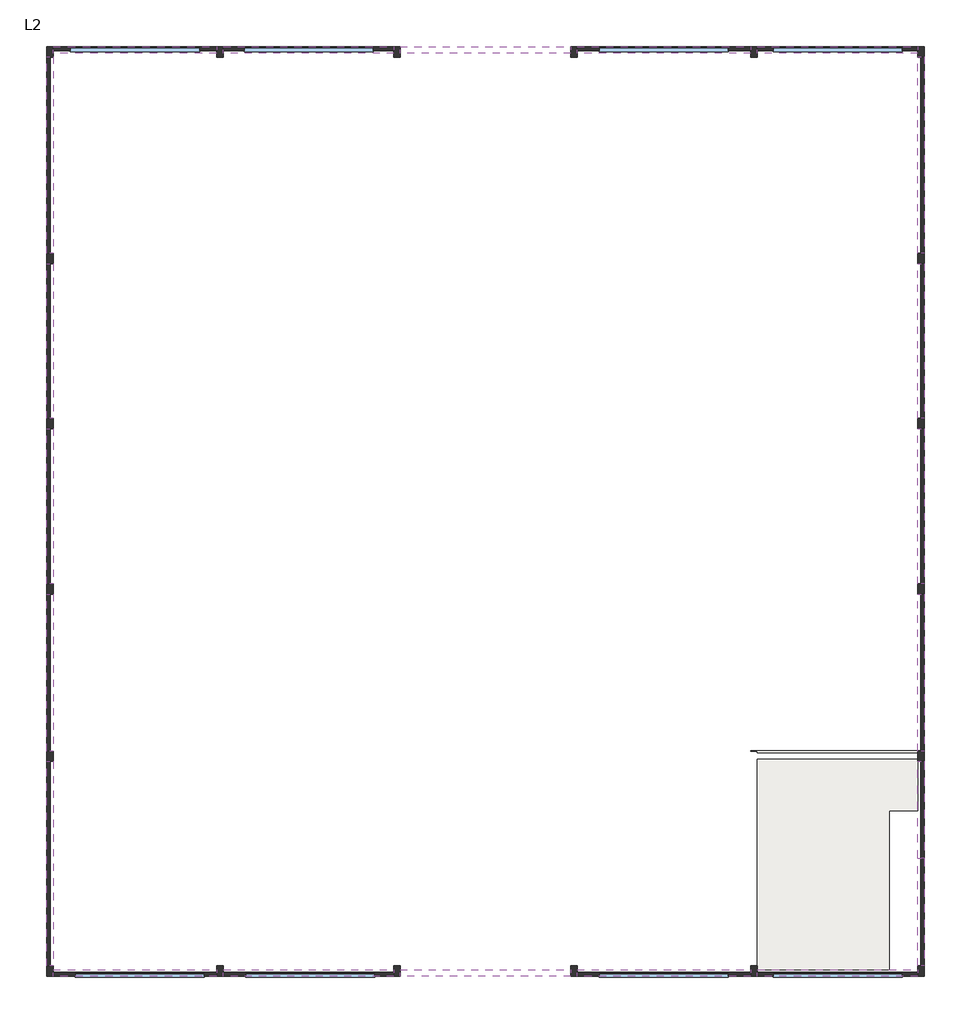
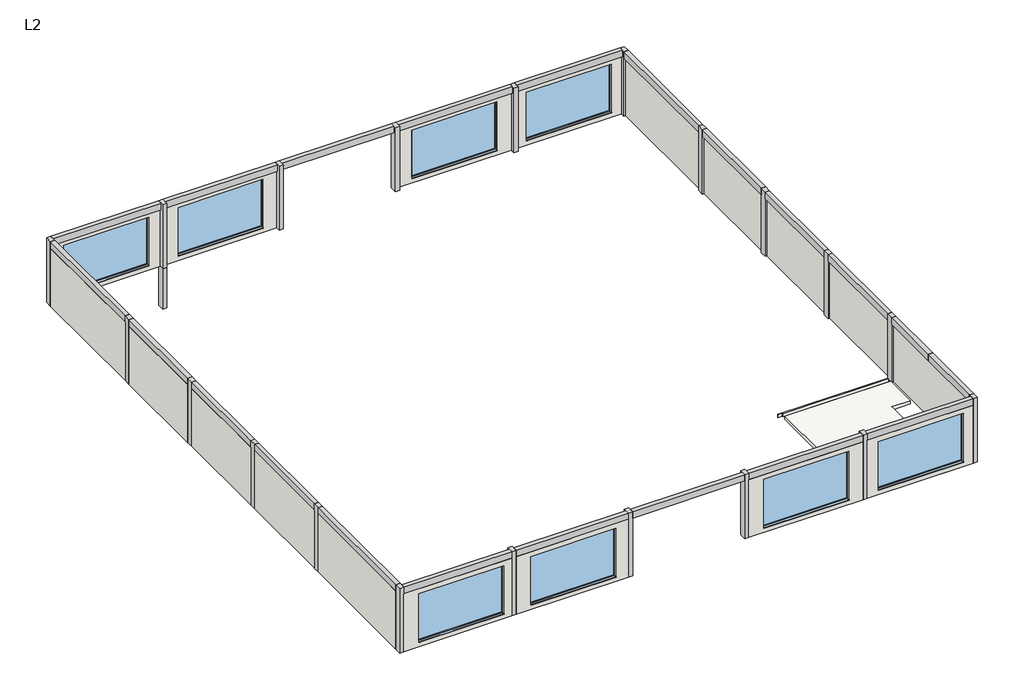
# One storey: 21 beams, 21 columns, 18 walls, 8 windows, 1 slab.
"""IFC4 building model written with IfcOpenShell, lengths in millimetres."""

import ifcopenshell
import ifcopenshell.guid

model = None  # the IFC model being written
_history = None  # IfcOwnerHistory: only IFC2X3 demands one
_inside = {}  # id of a spatial element -> (the spatial element, [elements in it])
_under = {}  # id of a project, library or spatial element -> (it, [spatial elements below it])
_declared = {}  # id of a project -> (the project, [libraries it declares])
_typed = {}  # id of a type object -> (the type object, [elements of that type])
_made_of = {}  # id of a material, layer set ... -> (it, [elements and type objects made of it])


def new_model(schema):
    """Start an empty IFC model of exactly this schema.

    Asked for "IFC4X3", IfcOpenShell would pick the latest addendum, in which some entities
    have other attributes; the version numbers below select the first issue.
    IFC2X3 requires an IfcOwnerHistory on every rooted entity: one is made here for all.
    """
    global model, _history
    if schema == "IFC4X3":
        model = ifcopenshell.file(schema_version=(4, 3, 0, 0))
    else:
        model = ifcopenshell.file(schema=schema)
    _inside.clear()
    _under.clear()
    _declared.clear()
    _typed.clear()
    _made_of.clear()
    _history = None
    if model.schema == "IFC2X3":
        org = make("IfcOrganization", Name="unknown")
        user = make(
            "IfcPersonAndOrganization",
            ThePerson=make("IfcPerson", FamilyName="unknown"),
            TheOrganization=org,
        )
        app = make(
            "IfcApplication",
            ApplicationDeveloper=org,
            Version="unknown",
            ApplicationFullName="unknown",
            ApplicationIdentifier="unknown",
        )
        _history = make(
            "IfcOwnerHistory",
            OwningUser=user,
            OwningApplication=app,
            ChangeAction="ADDED",
            CreationDate=0,
        )
    return model


def make(cls, **values):
    """One entity of the class cls with the attributes given. An attribute that is None is left unset."""
    return model.create_entity(
        cls, **{name: value for name, value in values.items() if value is not None}
    )


def rooted(cls, **values):
    """An entity with a GlobalId (a new one), such as an element, a storey or a relation."""
    return make(cls, GlobalId=ifcopenshell.guid.new(), OwnerHistory=_history, **values)


def si_unit(unit_type, name, prefix=None):
    """IfcSIUnit, for example si_unit("LENGTHUNIT", "METRE", prefix="MILLI")."""
    return make("IfcSIUnit", UnitType=unit_type, Prefix=prefix, Name=name)


def assignment(units):
    """IfcUnitAssignment: the units of a project."""
    return None if units is None else make("IfcUnitAssignment", Units=units)


def point(xyz):
    """IfcCartesianPoint."""
    return None if xyz is None else make("IfcCartesianPoint", Coordinates=xyz)


def direction(xyz):
    """IfcDirection."""
    return None if xyz is None else make("IfcDirection", DirectionRatios=xyz)


def frame(location, z_axis=None, x_axis=None):
    """IfcAxis2Placement3D, a coordinate frame: its origin and axes. An axis left out is left unset."""
    return make(
        "IfcAxis2Placement3D",
        Location=point(location),
        Axis=direction(z_axis),
        RefDirection=direction(x_axis),
    )


def origin():
    """The frame at (0, 0, 0) with its axes left unset."""
    return frame((0.0, 0.0, 0.0))


def place(relative_to, where):
    """IfcLocalPlacement: puts the frame where relative to a parent placement (None: the world)."""
    return make(
        "IfcLocalPlacement", PlacementRelTo=relative_to, RelativePlacement=where
    )


def context(
    kind, dimensions, precision=None, world=None, true_north=None, identifier=None
):
    """IfcGeometricRepresentationContext, for example the 3D "Model" context."""
    return make(
        "IfcGeometricRepresentationContext",
        ContextIdentifier=identifier,
        ContextType=kind,
        CoordinateSpaceDimension=dimensions,
        Precision=precision,
        WorldCoordinateSystem=world,
        TrueNorth=true_north,
    )


def project(units=None, contexts=None):
    """IfcProject with its units and contexts."""
    return rooted(
        "IfcProject",
        Name="project",
        RepresentationContexts=contexts,
        UnitsInContext=assignment(units),
    )


def spatial(cls, under=None, at=None, **own):
    """A site, building, storey or space (cls), placed at a placement, below another one or the project."""
    s = rooted(cls, ObjectPlacement=at, **own)
    if under is not None:
        _under.setdefault(under.id(), (under, []))[1].append(s)
    return s


def polyline(points):
    """IfcPolyline through the points."""
    return make("IfcPolyline", Points=[point(p) for p in points])


def outline(outer, holes=None, kind="AREA"):
    """IfcArbitraryClosedProfileDef: a profile drawn as a closed curve; with holes, ...WithVoids."""
    if holes is None:
        return make("IfcArbitraryClosedProfileDef", ProfileType=kind, OuterCurve=outer)
    return make(
        "IfcArbitraryProfileDefWithVoids",
        ProfileType=kind,
        OuterCurve=outer,
        InnerCurves=holes,
    )


def extrude(swept, where, along, depth):
    """IfcExtrudedAreaSolid: the profile swept, set in the frame where, extruded along a direction by depth."""
    return make(
        "IfcExtrudedAreaSolid",
        SweptArea=swept,
        Position=where,
        ExtrudedDirection=direction(along),
        Depth=depth,
    )


def faces_of(points, faces, orient=None, outer=None):
    """IfcFace entities. A face is a list of loops; a loop is a list of indices into points, from 0.

    orient and outer hold one flag for each loop. By default every Orientation is true, the
    first loop of a face is its IfcFaceOuterBound and the others are IfcFaceBound.
    """
    made = []
    for i, loops in enumerate(faces):
        bounds = []
        for j, loop in enumerate(loops):
            is_outer = j == 0 if outer is None else outer[i][j]
            bounds.append(
                make(
                    "IfcFaceOuterBound" if is_outer else "IfcFaceBound",
                    Bound=make("IfcPolyLoop", Polygon=[points[k] for k in loop]),
                    Orientation=True if orient is None else orient[i][j],
                )
            )
        made.append(make("IfcFace", Bounds=bounds))
    return made


def faceted_brep(points, faces, orient=None, outer=None, voids=None):
    """IfcFacetedBrep: a solid bounded by flat faces; with voids (closed shells), ...WithVoids."""
    shared = [point(p) for p in points]
    hull = make("IfcClosedShell", CfsFaces=faces_of(shared, faces, orient, outer))
    if voids is None:
        return make("IfcFacetedBrep", Outer=hull)
    return make(
        "IfcFacetedBrepWithVoids",
        Outer=hull,
        Voids=[
            make(cls, CfsFaces=faces_of(shared, fs, o, b)) for cls, fs, o, b in voids
        ],
    )


def shape(context_of_items, identifier, shape_type, items):
    """IfcShapeRepresentation: the items that make up one representation, for example the "Body"."""
    return make(
        "IfcShapeRepresentation",
        ContextOfItems=context_of_items,
        RepresentationIdentifier=identifier,
        RepresentationType=shape_type,
        Items=items,
    )


def source(mapping_origin, context_of_items, identifier, shape_type, items):
    """IfcRepresentationMap: a shape defined once, which mapped items show again and again."""
    return make(
        "IfcRepresentationMap",
        MappingOrigin=mapping_origin,
        MappedRepresentation=shape(context_of_items, identifier, shape_type, items),
    )


def transform(
    local_origin,
    x_axis=None,
    y_axis=None,
    z_axis=None,
    scale=None,
    scale2=None,
    scale3=None,
    uniform=True,
):
    """IfcCartesianTransformationOperator3D, or its non-uniform kind. x_axis, y_axis, z_axis: its Axis1, 2, 3."""
    if uniform:
        return make(
            "IfcCartesianTransformationOperator3D",
            Axis1=direction(x_axis),
            Axis2=direction(y_axis),
            LocalOrigin=point(local_origin),
            Scale=scale,
            Axis3=direction(z_axis),
        )
    return make(
        "IfcCartesianTransformationOperator3DnonUniform",
        Axis1=direction(x_axis),
        Axis2=direction(y_axis),
        LocalOrigin=point(local_origin),
        Scale=scale,
        Axis3=direction(z_axis),
        Scale2=scale2,
        Scale3=scale3,
    )


def mapped(mapping_source, mapping_target):
    """IfcMappedItem: shows the shape of a source again, moved by a transform."""
    return make(
        "IfcMappedItem", MappingSource=mapping_source, MappingTarget=mapping_target
    )


def made_of(thing, what):
    """Note that an element or type object is made of a material, layer set ...; save() writes the relation."""
    if what is not None:
        _made_of.setdefault(what.id(), (what, []))[1].append(thing)
    return thing


def element(
    cls,
    number,
    at=None,
    inside=None,
    cuts=None,
    type_object=None,
    material=None,
    context=None,
    identifier="Body",
    shape_type=None,
    held_by="IfcProductDefinitionShape",
    body=None,
    shapes=None,
    **own,
):
    """One element of the class cls, such as IfcWall. Its Tag is "e" and its number.

    at: its placement. inside: the storey or other place that contains it. cuts: it is an
    opening in that element (IfcRelVoidsElement). A single representation is given by context,
    identifier, shape_type and body (its items); several are given by shapes. held_by: the class
    of the entity that holds the representations. save() writes the other relations.
    """
    e = rooted(cls, Tag="e%d" % number, ObjectPlacement=at, **own)
    if body is not None:
        shapes = [shape(context, identifier, shape_type, body)]
    if shapes is not None:
        e.Representation = make(held_by, Representations=shapes)
    if inside is not None:
        _inside.setdefault(inside.id(), (inside, []))[1].append(e)
    if cuts is not None:
        rooted(
            "IfcRelVoidsElement", RelatingBuildingElement=cuts, RelatedOpeningElement=e
        )
    if type_object is not None:
        _typed.setdefault(type_object.id(), (type_object, []))[1].append(e)
    return made_of(e, material)


def aggregate(whole, parts):
    """IfcRelAggregates: a whole, such as a stair, and the parts it consists of."""
    return rooted("IfcRelAggregates", RelatingObject=whole, RelatedObjects=parts)


def save(model, path):
    """Write the relations noted so far, then the file.

    IfcRelAggregates (storeys below a building ...), IfcRelContainedInSpatialStructure (elements
    in a storey), IfcRelDefinesByType, IfcRelAssociatesMaterial and IfcRelDeclares: one each for
    every whole, place, type object, material and project.
    """
    for whole, parts in _under.values():
        aggregate(whole, parts)
    for where, things in _inside.values():
        rooted(
            "IfcRelContainedInSpatialStructure",
            RelatedElements=things,
            RelatingStructure=where,
        )
    for kind, things in _typed.values():
        rooted("IfcRelDefinesByType", RelatedObjects=things, RelatingType=kind)
    for what, things in _made_of.values():
        rooted("IfcRelAssociatesMaterial", RelatedObjects=things, RelatingMaterial=what)
    for by, libraries in _declared.values():
        rooted("IfcRelDeclares", RelatingContext=by, RelatedDefinitions=libraries)
    model.write(path)


def window_5000_x_3000mm_49c9fe68(model_context):
    return source(origin(), model_context, "Body", "SolidModel", [
        extrude(outline(polyline([(125.0, 920.0), (125.0, 900.0), (105.0, 900.0), (105.0, 910.0), (95.0, 910.0), (95.0, 900.0), (-25.0, 900.0), (-25.0, 920.0), (125.0, 920.0)])), frame((-2500.0, 0.0, 0.0), z_axis=(1.0, 0.0, 0.0), x_axis=(0.0, 1.0, 0.0)), (0.0, 0.0, 1.0), 5000.0),
        extrude(outline(polyline([(-2455.0, -49.0), (-2455.0, -35.0), (2455.0, -35.0), (2455.0, -49.0), (-2455.0, -49.0)])), frame((0.0, 0.0, 965.0), z_axis=(0.0, 0.0, 1.0), x_axis=(1.0, 0.0, 0.0)), (0.0, 0.0, 1.0), 2890.0),
        extrude(outline(polyline([(3865.0, -2465.0), (955.0, -2465.0), (955.0, 2465.0), (3865.0, 2465.0), (3865.0, -2465.0)]), holes=[polyline([(3840.0, 2440.0), (980.0, 2440.0), (980.0, -2440.0), (3840.0, -2440.0), (3840.0, 2440.0)])]), frame((0.0, -75.0, 0.0), z_axis=(0.0, 1.0, 0.0), x_axis=(0.0, 0.0, 1.0)), (0.0, 0.0, 1.0), 26.0),
        faceted_brep([(2500.0, -25.0, 3900.0), (2500.0, -75.0, 3900.0), (2500.0, -75.0, 900.0), (2500.0, -25.0, 900.0), (-2500.0, -75.0, 3900.0), (-2500.0, -75.0, 900.0), (-2465.0, -75.0, 3865.0), (2465.0, -75.0, 3865.0), (2465.0, -75.0, 955.0), (-2465.0, -75.0, 955.0), (-2500.0, -25.0, 900.0), (-2500.0, -25.0, 3900.0), (2440.0, -25.0, 3840.0), (-2440.0, -25.0, 3840.0), (-2440.0, -25.0, 980.0), (2440.0, -25.0, 980.0), (2440.0, -35.0, 3840.0), (2440.0, -35.0, 980.0), (-2440.0, -35.0, 980.0), (2465.0, -35.0, 3865.0), (-2465.0, -35.0, 3865.0), (-2465.0, -35.0, 955.0), (2465.0, -35.0, 955.0), (-2440.0, -35.0, 3840.0)], [[[0, 1, 2, 3]], [[2, 1, 4, 5], [6, 7, 8, 9]], [[5, 10, 3, 2]], [[10, 11, 0, 3], [12, 13, 14, 15]], [[16, 12, 15, 17]], [[17, 15, 14, 18]], [[19, 20, 21, 22], [23, 16, 17, 18]], [[7, 19, 22, 8]], [[8, 22, 21, 9]], [[13, 23, 18, 14]], [[20, 6, 9, 21]], [[4, 11, 10, 5]], [[11, 4, 1, 0]], [[23, 13, 12, 16]], [[6, 20, 19, 7]]]),
        extrude(outline(polyline([(3925.0, -2525.0), (875.0, -2525.0), (875.0, 2525.0), (3925.0, 2525.0), (3925.0, -2525.0)]), holes=[polyline([(3890.0, 2490.0), (910.0, 2490.0), (910.0, -2490.0), (3890.0, -2490.0), (3890.0, 2490.0)])]), frame((0.0, -80.0, 0.0), z_axis=(0.0, 1.0, 0.0), x_axis=(0.0, 0.0, 1.0)), (0.0, 0.0, 1.0), 5.0),
    ])


model = new_model("IFC4")

# Units and contexts
model_context = context("Model", 3, world=origin())
ifc_project = project(units=[si_unit("LENGTHUNIT", "METRE", prefix="MILLI")], contexts=[model_context])

# Site, building, storey
site = spatial("IfcSite", under=ifc_project)
building = spatial("IfcBuilding", under=site)
storey = spatial("IfcBuildingStorey", under=building, Name="L2", Elevation=4000.0)

# Beams
placement = place(None, origin())
element("IfcBeam", 1, ObjectType="M_Hormigón-Viga rectangular : 250 x 400mm", at=placement, inside=storey, context=model_context, shape_type="SweptSolid", body=[
    extrude(outline(polyline([(10525.0, 17750.0), (10525.0, 18000.0), (16750.0, 18000.0), (16750.0, 17750.0), (10525.0, 17750.0)])), frame((0.0, 0.0, 7600.0), z_axis=(0.0, 0.0, 1.0), x_axis=(1.0, 0.0, 0.0)), (0.0, 0.0, 1.0), 400.0),
])
element("IfcBeam", 2, ObjectType="M_Hormigón-Viga rectangular : 250 x 400mm", at=placement, inside=storey, context=model_context, shape_type="SweptSolid", body=[
    extrude(outline(polyline([(3550.0, 17750.0), (3550.0, 18000.0), (10275.0, 18000.0), (10275.0, 17750.0), (3550.0, 17750.0)])), frame((0.0, 0.0, 7600.0), z_axis=(0.0, 0.0, 1.0), x_axis=(1.0, 0.0, 0.0)), (0.0, 0.0, 1.0), 400.0),
])
element("IfcBeam", 3, ObjectType="M_Hormigón-Viga rectangular : 250 x 400mm", at=placement, inside=storey, context=model_context, shape_type="SweptSolid", body=[
    extrude(outline(polyline([(-3300.0, 17750.0), (-3300.0, 18000.0), (3300.0, 18000.0), (3300.0, 17750.0), (-3300.0, 17750.0)])), frame((0.0, 0.0, 7600.0), z_axis=(0.0, 0.0, 1.0), x_axis=(1.0, 0.0, 0.0)), (0.0, 0.0, 1.0), 400.0),
])
element("IfcBeam", 4, ObjectType="M_Hormigón-Viga rectangular : 250 x 400mm", at=placement, inside=storey, context=model_context, shape_type="SweptSolid", body=[
    extrude(outline(polyline([(-10150.0, 17750.0), (-10150.0, 18000.0), (-3550.0, 18000.0), (-3550.0, 17750.0), (-10150.0, 17750.0)])), frame((0.0, 0.0, 7600.0), z_axis=(0.0, 0.0, 1.0), x_axis=(1.0, 0.0, 0.0)), (0.0, 0.0, 1.0), 400.0),
])
element("IfcBeam", 5, ObjectType="M_Hormigón-Viga rectangular : 250 x 400mm", at=placement, inside=storey, context=model_context, shape_type="SweptSolid", body=[
    extrude(outline(polyline([(-16750.0, 17750.0), (-16750.0, 18000.0), (-10400.0, 18000.0), (-10400.0, 17750.0), (-16750.0, 17750.0)])), frame((0.0, 0.0, 7600.0), z_axis=(0.0, 0.0, 1.0), x_axis=(1.0, 0.0, 0.0)), (0.0, 0.0, 1.0), 400.0),
])
element("IfcBeam", 6, ObjectType="M_Hormigón-Viga rectangular : 250 x 400mm", at=placement, inside=storey, context=model_context, shape_type="SweptSolid", body=[
    extrude(outline(polyline([(16750.0, -17750.0), (16750.0, -18000.0), (10525.0, -18000.0), (10525.0, -17750.0), (16750.0, -17750.0)])), frame((0.0, 0.0, 7600.0), z_axis=(0.0, 0.0, 1.0), x_axis=(1.0, 0.0, 0.0)), (0.0, 0.0, 1.0), 400.0),
])
element("IfcBeam", 7, ObjectType="M_Hormigón-Viga rectangular : 250 x 400mm", at=placement, inside=storey, context=model_context, shape_type="SweptSolid", body=[
    extrude(outline(polyline([(10275.0, -17750.0), (10275.0, -18000.0), (3550.0, -18000.0), (3550.0, -17750.0), (10275.0, -17750.0)])), frame((0.0, 0.0, 7600.0), z_axis=(0.0, 0.0, 1.0), x_axis=(1.0, 0.0, 0.0)), (0.0, 0.0, 1.0), 400.0),
])
element("IfcBeam", 8, ObjectType="M_Hormigón-Viga rectangular : 250 x 400mm", at=placement, inside=storey, context=model_context, shape_type="SweptSolid", body=[
    extrude(outline(polyline([(3300.0, -17750.0), (3300.0, -18000.0), (-3300.0, -18000.0), (-3300.0, -17750.0), (3300.0, -17750.0)])), frame((0.0, 0.0, 7600.0), z_axis=(0.0, 0.0, 1.0), x_axis=(1.0, 0.0, 0.0)), (0.0, 0.0, 1.0), 400.0),
])
element("IfcBeam", 9, ObjectType="M_Hormigón-Viga rectangular : 250 x 400mm", at=placement, inside=storey, context=model_context, shape_type="SweptSolid", body=[
    extrude(outline(polyline([(-3550.0, -17750.0), (-3550.0, -18000.0), (-10150.0, -18000.0), (-10150.0, -17750.0), (-3550.0, -17750.0)])), frame((0.0, 0.0, 7600.0), z_axis=(0.0, 0.0, 1.0), x_axis=(1.0, 0.0, 0.0)), (0.0, 0.0, 1.0), 400.0),
])
element("IfcBeam", 10, ObjectType="M_Hormigón-Viga rectangular : 250 x 400mm", at=placement, inside=storey, context=model_context, shape_type="SweptSolid", body=[
    extrude(outline(polyline([(-10400.0, -17750.0), (-10400.0, -18000.0), (-16750.0, -18000.0), (-16750.0, -17750.0), (-10400.0, -17750.0)])), frame((0.0, 0.0, 7600.0), z_axis=(0.0, 0.0, 1.0), x_axis=(1.0, 0.0, 0.0)), (0.0, 0.0, 1.0), 400.0),
])
element("IfcBeam", 11, ObjectType="M_Hormigón-Viga rectangular : 250 x 400mm", at=placement, inside=storey, context=model_context, shape_type="SweptSolid", body=[
    extrude(outline(polyline([(-16750.0, -17600.0), (-17000.0, -17600.0), (-17000.0, -9685.0), (-16750.0, -9685.0), (-16750.0, -17600.0)])), frame((0.0, 0.0, 7600.0), z_axis=(0.0, 0.0, 1.0), x_axis=(1.0, 0.0, 0.0)), (0.0, 0.0, 1.0), 400.0),
])
element("IfcBeam", 12, ObjectType="M_Hormigón-Viga rectangular : 250 x 400mm", at=placement, inside=storey, context=model_context, shape_type="SweptSolid", body=[
    extrude(outline(polyline([(-16750.0, -9285.0), (-17000.0, -9285.0), (-17000.0, -3200.0), (-16750.0, -3200.0), (-16750.0, -9285.0)])), frame((0.0, 0.0, 7600.0), z_axis=(0.0, 0.0, 1.0), x_axis=(1.0, 0.0, 0.0)), (0.0, 0.0, 1.0), 400.0),
])
element("IfcBeam", 13, ObjectType="M_Hormigón-Viga rectangular : 250 x 400mm", at=placement, inside=storey, context=model_context, shape_type="SweptSolid", body=[
    extrude(outline(polyline([(-16750.0, -2800.0), (-17000.0, -2800.0), (-17000.0, 3200.0), (-16750.0, 3200.0), (-16750.0, -2800.0)])), frame((0.0, 0.0, 7600.0), z_axis=(0.0, 0.0, 1.0), x_axis=(1.0, 0.0, 0.0)), (0.0, 0.0, 1.0), 400.0),
])
element("IfcBeam", 14, ObjectType="M_Hormigón-Viga rectangular : 250 x 400mm", at=placement, inside=storey, context=model_context, shape_type="SweptSolid", body=[
    extrude(outline(polyline([(-16750.0, 3600.0), (-17000.0, 3600.0), (-17000.0, 9600.0), (-16750.0, 9600.0), (-16750.0, 3600.0)])), frame((0.0, 0.0, 7600.0), z_axis=(0.0, 0.0, 1.0), x_axis=(1.0, 0.0, 0.0)), (0.0, 0.0, 1.0), 400.0),
])
element("IfcBeam", 15, ObjectType="M_Hormigón-Viga rectangular : 250 x 400mm", at=placement, inside=storey, context=model_context, shape_type="SweptSolid", body=[
    extrude(outline(polyline([(-17000.0, 17600.0), (-16750.0, 17600.0), (-16750.0, 10000.0), (-17000.0, 10000.0), (-17000.0, 17600.0)])), frame((0.0, 0.0, 7600.0), z_axis=(0.0, 0.0, 1.0), x_axis=(1.0, 0.0, 0.0)), (0.0, 0.0, 1.0), 400.0),
])
element("IfcBeam", 16, ObjectType="M_Hormigón-Viga rectangular : 250 x 400mm", at=placement, inside=storey, context=model_context, shape_type="SweptSolid", body=[
    extrude(outline(polyline([(16750.0, -13440.5675387), (17000.0, -13440.5675387), (17000.0, -17600.0), (16750.0, -17600.0), (16750.0, -13440.5675387)])), frame((0.0, 0.0, 7600.0), z_axis=(0.0, 0.0, 1.0), x_axis=(1.0, 0.0, 0.0)), (0.0, 0.0, 1.0), 400.0),
])
element("IfcBeam", 17, ObjectType="M_Hormigón-Viga rectangular : 250 x 400mm", at=placement, inside=storey, context=model_context, shape_type="SweptSolid", body=[
    extrude(outline(polyline([(17000.0, -13440.5675387), (16750.0, -13440.5675387), (16750.0, -9685.0), (17000.0, -9685.0), (17000.0, -13440.5675387)])), frame((0.0, 0.0, 7600.0), z_axis=(0.0, 0.0, 1.0), x_axis=(1.0, 0.0, 0.0)), (0.0, 0.0, 1.0), 400.0),
])
element("IfcBeam", 18, ObjectType="M_Hormigón-Viga rectangular : 250 x 400mm", at=placement, inside=storey, context=model_context, shape_type="SweptSolid", body=[
    extrude(outline(polyline([(16750.0, -3200.0), (17000.0, -3200.0), (17000.0, -9285.0), (16750.0, -9285.0), (16750.0, -3200.0)])), frame((0.0, 0.0, 7600.0), z_axis=(0.0, 0.0, 1.0), x_axis=(1.0, 0.0, 0.0)), (0.0, 0.0, 1.0), 400.0),
])
element("IfcBeam", 19, ObjectType="M_Hormigón-Viga rectangular : 250 x 400mm", at=placement, inside=storey, context=model_context, shape_type="SweptSolid", body=[
    extrude(outline(polyline([(16750.0, 3200.0), (17000.0, 3200.0), (17000.0, -2800.0), (16750.0, -2800.0), (16750.0, 3200.0)])), frame((0.0, 0.0, 7600.0), z_axis=(0.0, 0.0, 1.0), x_axis=(1.0, 0.0, 0.0)), (0.0, 0.0, 1.0), 400.0),
])
element("IfcBeam", 20, ObjectType="M_Hormigón-Viga rectangular : 250 x 400mm", at=placement, inside=storey, context=model_context, shape_type="SweptSolid", body=[
    extrude(outline(polyline([(16750.0, 9600.0), (17000.0, 9600.0), (17000.0, 3600.0), (16750.0, 3600.0), (16750.0, 9600.0)])), frame((0.0, 0.0, 7600.0), z_axis=(0.0, 0.0, 1.0), x_axis=(1.0, 0.0, 0.0)), (0.0, 0.0, 1.0), 400.0),
])
element("IfcBeam", 21, ObjectType="M_Hormigón-Viga rectangular : 250 x 400mm", at=placement, inside=storey, context=model_context, shape_type="SweptSolid", body=[
    extrude(outline(polyline([(16750.0, 17600.0), (17000.0, 17600.0), (17000.0, 10000.0), (16750.0, 10000.0), (16750.0, 17600.0)])), frame((0.0, 0.0, 7600.0), z_axis=(0.0, 0.0, 1.0), x_axis=(1.0, 0.0, 0.0)), (0.0, 0.0, 1.0), 400.0),
])

# Columns
element("IfcColumn", 22, ObjectType="M_Hormigón-Rectangular-Pilar : 250 x 400mm", at=placement, inside=storey, context=model_context, shape_type="Brep", body=[
    faceted_brep([(-10150.0, 18000.0, 1500.0), (-10150.0, 17600.0, 1500.0), (-10400.0, 17600.0, 1500.0), (-10400.0, 18000.0, 1500.0), (-10150.0, 18000.0, 4000.0), (-10150.0, 17750.0, 4000.0), (-10150.0, 17600.0, 4000.0), (-10150.0, 18000.0, 3600.0), (-10400.0, 17600.0, 4000.0), (-10400.0, 17750.0, 4000.0), (-10400.0, 18000.0, 4000.0), (-10400.0, 18000.0, 3600.0)], [[[0, 1, 2, 3]], [[4, 5, 6, 1, 0, 7]], [[6, 8, 2, 1]], [[8, 9, 10, 11, 3, 2]], [[10, 4, 7, 0, 3, 11]], [[4, 10, 9, 8, 6, 5]]]),
])
element("IfcColumn", 23, ObjectType="M_Hormigón-Rectangular-Pilar : 250 x 400mm", at=placement, inside=storey, context=model_context, shape_type="SweptSolid", body=[
    extrude(outline(polyline([(-16750.0, 18000.0), (-16750.0, 17600.0), (-17000.0, 17600.0), (-17000.0, 18000.0), (-16750.0, 18000.0)])), frame((0.0, 0.0, 4000.0), z_axis=(0.0, 0.0, 1.0), x_axis=(1.0, 0.0, 0.0)), (0.0, 0.0, 1.0), 4000.0),
])
element("IfcColumn", 24, ObjectType="M_Hormigón-Rectangular-Pilar : 250 x 400mm", at=placement, inside=storey, context=model_context, shape_type="SweptSolid", body=[
    extrude(outline(polyline([(-10150.0, 18000.0), (-10150.0, 17600.0), (-10400.0, 17600.0), (-10400.0, 18000.0), (-10150.0, 18000.0)])), frame((0.0, 0.0, 4000.0), z_axis=(0.0, 0.0, 1.0), x_axis=(1.0, 0.0, 0.0)), (0.0, 0.0, 1.0), 4000.0),
])
element("IfcColumn", 25, ObjectType="M_Hormigón-Rectangular-Pilar : 250 x 400mm", at=placement, inside=storey, context=model_context, shape_type="SweptSolid", body=[
    extrude(outline(polyline([(-3300.0, 18000.0), (-3300.0, 17600.0), (-3550.0, 17600.0), (-3550.0, 18000.0), (-3300.0, 18000.0)])), frame((0.0, 0.0, 4000.0), z_axis=(0.0, 0.0, 1.0), x_axis=(1.0, 0.0, 0.0)), (0.0, 0.0, 1.0), 4000.0),
])
element("IfcColumn", 26, ObjectType="M_Hormigón-Rectangular-Pilar : 250 x 400mm", at=placement, inside=storey, context=model_context, shape_type="SweptSolid", body=[
    extrude(outline(polyline([(3550.0, 18000.0), (3550.0, 17600.0), (3300.0, 17600.0), (3300.0, 18000.0), (3550.0, 18000.0)])), frame((0.0, 0.0, 4000.0), z_axis=(0.0, 0.0, 1.0), x_axis=(1.0, 0.0, 0.0)), (0.0, 0.0, 1.0), 4000.0),
])
element("IfcColumn", 27, ObjectType="M_Hormigón-Rectangular-Pilar : 250 x 400mm", at=placement, inside=storey, context=model_context, shape_type="SweptSolid", body=[
    extrude(outline(polyline([(10525.0, 18000.0), (10525.0, 17600.0), (10275.0, 17600.0), (10275.0, 18000.0), (10525.0, 18000.0)])), frame((0.0, 0.0, 4000.0), z_axis=(0.0, 0.0, 1.0), x_axis=(1.0, 0.0, 0.0)), (0.0, 0.0, 1.0), 4000.0),
])
element("IfcColumn", 28, ObjectType="M_Hormigón-Rectangular-Pilar : 250 x 400mm", at=placement, inside=storey, context=model_context, shape_type="SweptSolid", body=[
    extrude(outline(polyline([(17000.0, 18000.0), (17000.0, 17600.0), (16750.0, 17600.0), (16750.0, 18000.0), (17000.0, 18000.0)])), frame((0.0, 0.0, 4000.0), z_axis=(0.0, 0.0, 1.0), x_axis=(1.0, 0.0, 0.0)), (0.0, 0.0, 1.0), 4000.0),
])
element("IfcColumn", 29, ObjectType="M_Hormigón-Rectangular-Pilar : 250 x 400mm", at=placement, inside=storey, context=model_context, shape_type="SweptSolid", body=[
    extrude(outline(polyline([(17000.0, 10000.0), (17000.0, 9600.0), (16750.0, 9600.0), (16750.0, 10000.0), (17000.0, 10000.0)])), frame((0.0, 0.0, 4000.0), z_axis=(0.0, 0.0, 1.0), x_axis=(1.0, 0.0, 0.0)), (0.0, 0.0, 1.0), 4000.0),
])
element("IfcColumn", 30, ObjectType="M_Hormigón-Rectangular-Pilar : 250 x 400mm", at=placement, inside=storey, context=model_context, shape_type="SweptSolid", body=[
    extrude(outline(polyline([(17000.0, 3600.0), (17000.0, 3200.0), (16750.0, 3200.0), (16750.0, 3600.0), (17000.0, 3600.0)])), frame((0.0, 0.0, 4000.0), z_axis=(0.0, 0.0, 1.0), x_axis=(1.0, 0.0, 0.0)), (0.0, 0.0, 1.0), 4000.0),
])
element("IfcColumn", 31, ObjectType="M_Hormigón-Rectangular-Pilar : 250 x 400mm", at=placement, inside=storey, context=model_context, shape_type="SweptSolid", body=[
    extrude(outline(polyline([(17000.0, -2800.0), (17000.0, -3200.0), (16750.0, -3200.0), (16750.0, -2800.0), (17000.0, -2800.0)])), frame((0.0, 0.0, 4000.0), z_axis=(0.0, 0.0, 1.0), x_axis=(1.0, 0.0, 0.0)), (0.0, 0.0, 1.0), 4000.0),
])
element("IfcColumn", 32, ObjectType="M_Hormigón-Rectangular-Pilar : 250 x 400mm", at=placement, inside=storey, context=model_context, shape_type="SweptSolid", body=[
    extrude(outline(polyline([(17000.0, -9285.0), (17000.0, -9685.0), (16750.0, -9685.0), (16750.0, -9285.0), (17000.0, -9285.0)])), frame((0.0, 0.0, 4000.0), z_axis=(0.0, 0.0, 1.0), x_axis=(1.0, 0.0, 0.0)), (0.0, 0.0, 1.0), 4000.0),
])
element("IfcColumn", 33, ObjectType="M_Hormigón-Rectangular-Pilar : 250 x 400mm", at=placement, inside=storey, context=model_context, shape_type="SweptSolid", body=[
    extrude(outline(polyline([(17000.0, -17600.0), (17000.0, -18000.0), (16750.0, -18000.0), (16750.0, -17600.0), (17000.0, -17600.0)])), frame((0.0, 0.0, 4000.0), z_axis=(0.0, 0.0, 1.0), x_axis=(1.0, 0.0, 0.0)), (0.0, 0.0, 1.0), 4000.0),
])
element("IfcColumn", 34, ObjectType="M_Hormigón-Rectangular-Pilar : 250 x 400mm", at=placement, inside=storey, context=model_context, shape_type="SweptSolid", body=[
    extrude(outline(polyline([(10525.0, -17600.0), (10525.0, -18000.0), (10275.0, -18000.0), (10275.0, -17600.0), (10525.0, -17600.0)])), frame((0.0, 0.0, 4000.0), z_axis=(0.0, 0.0, 1.0), x_axis=(1.0, 0.0, 0.0)), (0.0, 0.0, 1.0), 4000.0),
])
element("IfcColumn", 35, ObjectType="M_Hormigón-Rectangular-Pilar : 250 x 400mm", at=placement, inside=storey, context=model_context, shape_type="SweptSolid", body=[
    extrude(outline(polyline([(3550.0, -17600.0), (3550.0, -18000.0), (3300.0, -18000.0), (3300.0, -17600.0), (3550.0, -17600.0)])), frame((0.0, 0.0, 4000.0), z_axis=(0.0, 0.0, 1.0), x_axis=(1.0, 0.0, 0.0)), (0.0, 0.0, 1.0), 4000.0),
])
element("IfcColumn", 36, ObjectType="M_Hormigón-Rectangular-Pilar : 250 x 400mm", at=placement, inside=storey, context=model_context, shape_type="SweptSolid", body=[
    extrude(outline(polyline([(-3300.0, -17600.0), (-3300.0, -18000.0), (-3550.0, -18000.0), (-3550.0, -17600.0), (-3300.0, -17600.0)])), frame((0.0, 0.0, 4000.0), z_axis=(0.0, 0.0, 1.0), x_axis=(1.0, 0.0, 0.0)), (0.0, 0.0, 1.0), 4000.0),
])
element("IfcColumn", 37, ObjectType="M_Hormigón-Rectangular-Pilar : 250 x 400mm", at=placement, inside=storey, context=model_context, shape_type="SweptSolid", body=[
    extrude(outline(polyline([(-10150.0, -17600.0), (-10150.0, -18000.0), (-10400.0, -18000.0), (-10400.0, -17600.0), (-10150.0, -17600.0)])), frame((0.0, 0.0, 4000.0), z_axis=(0.0, 0.0, 1.0), x_axis=(1.0, 0.0, 0.0)), (0.0, 0.0, 1.0), 4000.0),
])
element("IfcColumn", 38, ObjectType="M_Hormigón-Rectangular-Pilar : 250 x 400mm", at=placement, inside=storey, context=model_context, shape_type="SweptSolid", body=[
    extrude(outline(polyline([(-16750.0, -17600.0), (-16750.0, -18000.0), (-17000.0, -18000.0), (-17000.0, -17600.0), (-16750.0, -17600.0)])), frame((0.0, 0.0, 4000.0), z_axis=(0.0, 0.0, 1.0), x_axis=(1.0, 0.0, 0.0)), (0.0, 0.0, 1.0), 4000.0),
])
element("IfcColumn", 39, ObjectType="M_Hormigón-Rectangular-Pilar : 250 x 400mm", at=placement, inside=storey, context=model_context, shape_type="SweptSolid", body=[
    extrude(outline(polyline([(-16750.0, -9285.0), (-16750.0, -9685.0), (-17000.0, -9685.0), (-17000.0, -9285.0), (-16750.0, -9285.0)])), frame((0.0, 0.0, 4000.0), z_axis=(0.0, 0.0, 1.0), x_axis=(1.0, 0.0, 0.0)), (0.0, 0.0, 1.0), 4000.0),
])
element("IfcColumn", 40, ObjectType="M_Hormigón-Rectangular-Pilar : 250 x 400mm", at=placement, inside=storey, context=model_context, shape_type="SweptSolid", body=[
    extrude(outline(polyline([(-16750.0, -2800.0), (-16750.0, -3200.0), (-17000.0, -3200.0), (-17000.0, -2800.0), (-16750.0, -2800.0)])), frame((0.0, 0.0, 4000.0), z_axis=(0.0, 0.0, 1.0), x_axis=(1.0, 0.0, 0.0)), (0.0, 0.0, 1.0), 4000.0),
])
element("IfcColumn", 41, ObjectType="M_Hormigón-Rectangular-Pilar : 250 x 400mm", at=placement, inside=storey, context=model_context, shape_type="SweptSolid", body=[
    extrude(outline(polyline([(-16750.0, 3600.0), (-16750.0, 3200.0), (-17000.0, 3200.0), (-17000.0, 3600.0), (-16750.0, 3600.0)])), frame((0.0, 0.0, 4000.0), z_axis=(0.0, 0.0, 1.0), x_axis=(1.0, 0.0, 0.0)), (0.0, 0.0, 1.0), 4000.0),
])
element("IfcColumn", 42, ObjectType="M_Hormigón-Rectangular-Pilar : 250 x 400mm", at=placement, inside=storey, context=model_context, shape_type="SweptSolid", body=[
    extrude(outline(polyline([(-16750.0, 10000.0), (-16750.0, 9600.0), (-17000.0, 9600.0), (-17000.0, 10000.0), (-16750.0, 10000.0)])), frame((0.0, 0.0, 4000.0), z_axis=(0.0, 0.0, 1.0), x_axis=(1.0, 0.0, 0.0)), (0.0, 0.0, 1.0), 4000.0),
])

# Slab
element("IfcSlab", 43, ObjectType="Genérico 200 mm", at=placement, inside=storey, context=model_context, shape_type="Brep", body=[
    faceted_brep([(16750.0, -9595.0, 3800.0), (16750.0, -11597.1858803, 3800.0), (15647.5726879, -11597.1858803, 3800.0), (15647.5726879, -16650.0764278, 3800.0), (15647.5726879, -17750.0, 3800.0), (10525.0, -17750.0, 3800.0), (10525.0, -9595.0, 3800.0), (15647.5726879, -11597.1858803, 4000.0), (16750.0, -11597.1858803, 4000.0), (16750.0, -9685.0, 4000.0), (16750.0, -9595.0, 4000.0), (10525.0, -9595.0, 4000.0), (10525.0, -9685.0, 4000.0), (10525.0, -13240.5675387, 4000.0), (10525.0, -13640.5675387, 4000.0), (10525.0, -17600.0, 4000.0), (10525.0, -17750.0, 4000.0), (15647.5726879, -17750.0, 4000.0), (15647.5726879, -16650.0764278, 4000.0)], [[[0, 1, 2, 3, 4, 5, 6]], [[7, 8, 9, 10, 11, 12, 13, 14, 15, 16, 17, 18]], [[2, 1, 8, 7]], [[3, 2, 7, 18]], [[4, 3, 18, 17]], [[11, 6, 5, 16, 15, 14, 13, 12]], [[0, 10, 9, 8, 1]], [[0, 6, 11, 10]], [[5, 4, 17, 16]]]),
    faceted_brep([(10275.0, -9270.0, 3800.0), (16750.0, -9270.0, 3800.0), (17000.0, -9270.0, 3800.0), (17000.0, -9285.0, 3800.0), (16750.0, -9285.0, 3800.0), (16750.0, -9345.0, 3800.0), (10525.0, -9345.0, 3800.0), (10525.0, -9285.0, 3800.0), (10275.0, -9285.0, 3800.0), (17000.0, -9270.0, 4000.0), (16750.0, -9270.0, 4000.0), (10275.0, -9270.0, 4000.0), (10275.0, -9285.0, 4000.0), (10525.0, -9285.0, 4000.0), (10525.0, -9345.0, 4000.0), (16750.0, -9345.0, 4000.0), (16750.0, -9285.0, 4000.0), (17000.0, -9285.0, 4000.0)], [[[0, 1, 2, 3, 4, 5, 6, 7, 8]], [[9, 10, 11, 12, 13, 14, 15, 16, 17]], [[2, 9, 17, 3]], [[11, 0, 8, 12]], [[2, 1, 0, 11, 10, 9]], [[7, 13, 12, 8]], [[13, 7, 6, 14]], [[4, 16, 15, 5]], [[16, 4, 3, 17]], [[6, 5, 15, 14]]]),
])

# Walls
element("IfcWall", 44, ObjectType="Genérico - 150 mm DAPC", at=placement, inside=storey, context=model_context, shape_type="SweptSolid", body=[
    extrude(outline(polyline([(4000.0, -16750.0), (4000.0, -10400.0), (7600.0, -10400.0), (7600.0, -16750.0), (4000.0, -16750.0)]), holes=[polyline([(4300.0, -10887.5), (4300.0, -15887.5), (7300.0, -15887.5), (7300.0, -10887.5), (4300.0, -10887.5)])]), frame((0.0, -18000.0, 0.0), z_axis=(0.0, 1.0, 0.0), x_axis=(0.0, 0.0, 1.0)), (0.0, 0.0, 1.0), 150.0),
])
element("IfcWall", 45, ObjectType="Genérico - 150 mm DAPC", at=placement, inside=storey, context=model_context, shape_type="SweptSolid", body=[
    extrude(outline(polyline([(4000.0, -10150.0), (4000.0, -3550.0), (7600.0, -3550.0), (7600.0, -10150.0), (4000.0, -10150.0)]), holes=[polyline([(4300.0, -4287.5), (4300.0, -9287.5), (7300.0, -9287.5), (7300.0, -4287.5), (4300.0, -4287.5)])]), frame((0.0, -18000.0, 0.0), z_axis=(0.0, 1.0, 0.0), x_axis=(0.0, 0.0, 1.0)), (0.0, 0.0, 1.0), 150.0),
])
element("IfcWall", 46, ObjectType="Genérico - 150 mm DAPC", at=placement, inside=storey, context=model_context, shape_type="SweptSolid", body=[
    extrude(outline(polyline([(4000.0, 3550.0), (4000.0, 10275.0), (7600.0, 10275.0), (7600.0, 3550.0), (4000.0, 3550.0)]), holes=[polyline([(7300.0, 9412.5), (4300.0, 9412.5), (4300.0, 4412.5), (7300.0, 4412.5), (7300.0, 9412.5)])]), frame((0.0, -18000.0, 0.0), z_axis=(0.0, 1.0, 0.0), x_axis=(0.0, 0.0, 1.0)), (0.0, 0.0, 1.0), 150.0),
])
element("IfcWall", 47, ObjectType="Genérico - 150 mm DAPC", at=placement, inside=storey, context=model_context, shape_type="SweptSolid", body=[
    extrude(outline(polyline([(4000.0, 10525.0), (4000.0, 16750.0), (7600.0, 16750.0), (7600.0, 10525.0), (4000.0, 10525.0)]), holes=[polyline([(4300.0, 16150.0), (4300.0, 11150.0), (7300.0, 11150.0), (7300.0, 16150.0), (4300.0, 16150.0)])]), frame((0.0, -18000.0, 0.0), z_axis=(0.0, 1.0, 0.0), x_axis=(0.0, 0.0, 1.0)), (0.0, 0.0, 1.0), 150.0),
])
element("IfcWall", 48, ObjectType="Genérico - 150 mm DAPC", at=placement, inside=storey, context=model_context, shape_type="SweptSolid", body=[
    extrude(outline(polyline([(17000.0, -9670.0), (17000.0, -17600.0), (16850.0, -17600.0), (16850.0, -9670.0), (17000.0, -9670.0)])), frame((0.0, 0.0, 4000.0), z_axis=(0.0, 0.0, 1.0), x_axis=(1.0, 0.0, 0.0)), (0.0, 0.0, 1.0), 3600.0),
])
element("IfcWall", 49, ObjectType="Genérico - 150 mm DAPC", at=placement, inside=storey, context=model_context, shape_type="SweptSolid", body=[
    extrude(outline(polyline([(17000.0, -3200.0), (17000.0, -9270.0), (16850.0, -9270.0), (16850.0, -3200.0), (17000.0, -3200.0)])), frame((0.0, 0.0, 4000.0), z_axis=(0.0, 0.0, 1.0), x_axis=(1.0, 0.0, 0.0)), (0.0, 0.0, 1.0), 3600.0),
])
element("IfcWall", 50, ObjectType="Genérico - 150 mm DAPC", at=placement, inside=storey, context=model_context, shape_type="SweptSolid", body=[
    extrude(outline(polyline([(17000.0, 3200.0), (17000.0, -2800.0), (16850.0, -2800.0), (16850.0, 3200.0), (17000.0, 3200.0)])), frame((0.0, 0.0, 4000.0), z_axis=(0.0, 0.0, 1.0), x_axis=(1.0, 0.0, 0.0)), (0.0, 0.0, 1.0), 3600.0),
])
element("IfcWall", 51, ObjectType="Genérico - 150 mm DAPC", at=placement, inside=storey, context=model_context, shape_type="SweptSolid", body=[
    extrude(outline(polyline([(17000.0, 9600.0), (17000.0, 3600.0), (16850.0, 3600.0), (16850.0, 9600.0), (17000.0, 9600.0)])), frame((0.0, 0.0, 4000.0), z_axis=(0.0, 0.0, 1.0), x_axis=(1.0, 0.0, 0.0)), (0.0, 0.0, 1.0), 3600.0),
])
element("IfcWall", 52, ObjectType="Genérico - 150 mm DAPC", at=placement, inside=storey, context=model_context, shape_type="SweptSolid", body=[
    extrude(outline(polyline([(17000.0, 17600.0), (17000.0, 10000.0), (16850.0, 10000.0), (16850.0, 17600.0), (17000.0, 17600.0)])), frame((0.0, 0.0, 4000.0), z_axis=(0.0, 0.0, 1.0), x_axis=(1.0, 0.0, 0.0)), (0.0, 0.0, 1.0), 3600.0),
])
element("IfcWall", 53, ObjectType="Genérico - 150 mm DAPC", at=placement, inside=storey, context=model_context, shape_type="SweptSolid", body=[
    extrude(outline(polyline([(4000.0, 10525.0), (4000.0, 16750.0), (7600.0, 16750.0), (7600.0, 10525.0), (4000.0, 10525.0)]), holes=[polyline([(7300.0, 16137.5), (4300.0, 16137.5), (4300.0, 11137.5), (7300.0, 11137.5), (7300.0, 16137.5)])]), frame((0.0, 17850.0, 0.0), z_axis=(0.0, 1.0, 0.0), x_axis=(0.0, 0.0, 1.0)), (0.0, 0.0, 1.0), 150.0),
])
element("IfcWall", 54, ObjectType="Genérico - 150 mm DAPC", at=placement, inside=storey, context=model_context, shape_type="SweptSolid", body=[
    extrude(outline(polyline([(4000.0, 3550.0), (4000.0, 10275.0), (7600.0, 10275.0), (7600.0, 3550.0), (4000.0, 3550.0)]), holes=[polyline([(7300.0, 9412.5), (4300.0, 9412.5), (4300.0, 4412.5), (7300.0, 4412.5), (7300.0, 9412.5)])]), frame((0.0, 17850.0, 0.0), z_axis=(0.0, 1.0, 0.0), x_axis=(0.0, 0.0, 1.0)), (0.0, 0.0, 1.0), 150.0),
])
element("IfcWall", 55, ObjectType="Genérico - 150 mm DAPC", at=placement, inside=storey, context=model_context, shape_type="SweptSolid", body=[
    extrude(outline(polyline([(4000.0, -10150.0), (4000.0, -3550.0), (7600.0, -3550.0), (7600.0, -10150.0), (4000.0, -10150.0)]), holes=[polyline([(7300.0, -4350.0), (4300.0, -4350.0), (4300.0, -9350.0), (7300.0, -9350.0), (7300.0, -4350.0)])]), frame((0.0, 17850.0, 0.0), z_axis=(0.0, 1.0, 0.0), x_axis=(0.0, 0.0, 1.0)), (0.0, 0.0, 1.0), 150.0),
])
element("IfcWall", 56, ObjectType="Genérico - 150 mm DAPC", at=placement, inside=storey, context=model_context, shape_type="SweptSolid", body=[
    extrude(outline(polyline([(4000.0, -16750.0), (4000.0, -10400.0), (7600.0, -10400.0), (7600.0, -16750.0), (4000.0, -16750.0)]), holes=[polyline([(7300.0, -11075.0), (4300.0, -11075.0), (4300.0, -16075.0), (7300.0, -16075.0), (7300.0, -11075.0)])]), frame((0.0, 17850.0, 0.0), z_axis=(0.0, 1.0, 0.0), x_axis=(0.0, 0.0, 1.0)), (0.0, 0.0, 1.0), 150.0),
])
element("IfcWall", 57, ObjectType="Genérico - 150 mm DAPC", at=placement, inside=storey, context=model_context, shape_type="SweptSolid", body=[
    extrude(outline(polyline([(-17000.0, 10000.0), (-17000.0, 17600.0), (-16850.0, 17600.0), (-16850.0, 10000.0), (-17000.0, 10000.0)])), frame((0.0, 0.0, 4000.0), z_axis=(0.0, 0.0, 1.0), x_axis=(1.0, 0.0, 0.0)), (0.0, 0.0, 1.0), 3600.0),
])
element("IfcWall", 58, ObjectType="Genérico - 150 mm DAPC", at=placement, inside=storey, context=model_context, shape_type="SweptSolid", body=[
    extrude(outline(polyline([(-17000.0, 3600.0), (-17000.0, 9600.0), (-16850.0, 9600.0), (-16850.0, 3600.0), (-17000.0, 3600.0)])), frame((0.0, 0.0, 4000.0), z_axis=(0.0, 0.0, 1.0), x_axis=(1.0, 0.0, 0.0)), (0.0, 0.0, 1.0), 3600.0),
])
element("IfcWall", 59, ObjectType="Genérico - 150 mm DAPC", at=placement, inside=storey, context=model_context, shape_type="SweptSolid", body=[
    extrude(outline(polyline([(-17000.0, -2800.0), (-17000.0, 3200.0), (-16850.0, 3200.0), (-16850.0, -2800.0), (-17000.0, -2800.0)])), frame((0.0, 0.0, 4000.0), z_axis=(0.0, 0.0, 1.0), x_axis=(1.0, 0.0, 0.0)), (0.0, 0.0, 1.0), 3600.0),
])
element("IfcWall", 60, ObjectType="Genérico - 150 mm DAPC", at=placement, inside=storey, context=model_context, shape_type="SweptSolid", body=[
    extrude(outline(polyline([(-17000.0, -9270.0), (-17000.0, -3200.0), (-16850.0, -3200.0), (-16850.0, -9270.0), (-17000.0, -9270.0)])), frame((0.0, 0.0, 4000.0), z_axis=(0.0, 0.0, 1.0), x_axis=(1.0, 0.0, 0.0)), (0.0, 0.0, 1.0), 3600.0),
])
element("IfcWall", 61, ObjectType="Genérico - 150 mm DAPC", at=placement, inside=storey, context=model_context, shape_type="SweptSolid", body=[
    extrude(outline(polyline([(-17000.0, -17600.0), (-17000.0, -9670.0), (-16850.0, -9670.0), (-16850.0, -17600.0), (-17000.0, -17600.0)])), frame((0.0, 0.0, 4000.0), z_axis=(0.0, 0.0, 1.0), x_axis=(1.0, 0.0, 0.0)), (0.0, 0.0, 1.0), 3600.0),
])

# Windows
window_5000_x_3000mm_shape = window_5000_x_3000mm_49c9fe68(model_context)
element("IfcWindow", 62, ObjectType="Ventana simple fija con cubrejuntas interior : 5000 x 3000mm", at=placement, inside=storey, context=model_context, shape_type="MappedRepresentation", body=[
    mapped(window_5000_x_3000mm_shape, transform((6912.5, -17925.0, 3400.0), x_axis=(-1.0, 0.0, 0.0), y_axis=(0.0, -1.0, 0.0), z_axis=(0.0, 0.0, 1.0))),
])
element("IfcWindow", 63, ObjectType="Ventana simple fija con cubrejuntas interior : 5000 x 3000mm", at=placement, inside=storey, context=model_context, shape_type="MappedRepresentation", body=[
    mapped(window_5000_x_3000mm_shape, transform((13650.0, -17925.0, 3400.0), x_axis=(-1.0, 0.0, 0.0), y_axis=(0.0, -1.0, 0.0), z_axis=(0.0, 0.0, 1.0))),
])
element("IfcWindow", 64, ObjectType="Ventana simple fija con cubrejuntas interior : 5000 x 3000mm", at=placement, inside=storey, context=model_context, shape_type="MappedRepresentation", body=[
    mapped(window_5000_x_3000mm_shape, transform((-6787.5, -17925.0, 3400.0), x_axis=(-1.0, 0.0, 0.0), y_axis=(0.0, -1.0, 0.0), z_axis=(0.0, 0.0, 1.0))),
])
element("IfcWindow", 65, ObjectType="Ventana simple fija con cubrejuntas interior : 5000 x 3000mm", at=placement, inside=storey, context=model_context, shape_type="MappedRepresentation", body=[
    mapped(window_5000_x_3000mm_shape, transform((-13387.5, -17925.0, 3400.0), x_axis=(-1.0, 0.0, 0.0), y_axis=(0.0, -1.0, 0.0), z_axis=(0.0, 0.0, 1.0))),
])
element("IfcWindow", 66, ObjectType="Ventana simple fija con cubrejuntas interior : 5000 x 3000mm", at=placement, inside=storey, context=model_context, shape_type="MappedRepresentation", body=[
    mapped(window_5000_x_3000mm_shape, transform((-13575.0, 17925.0, 3400.0), x_axis=(-1.0, 0.0, 0.0), y_axis=(0.0, -1.0, 0.0), z_axis=(0.0, 0.0, 1.0))),
])
element("IfcWindow", 67, ObjectType="Ventana simple fija con cubrejuntas interior : 5000 x 3000mm", at=placement, inside=storey, context=model_context, shape_type="MappedRepresentation", body=[
    mapped(window_5000_x_3000mm_shape, transform((-6850.0, 17925.0, 3400.0), x_axis=(-1.0, 0.0, 0.0), y_axis=(0.0, -1.0, 0.0), z_axis=(0.0, 0.0, 1.0))),
])
element("IfcWindow", 68, ObjectType="Ventana simple fija con cubrejuntas interior : 5000 x 3000mm", at=placement, inside=storey, context=model_context, shape_type="MappedRepresentation", body=[
    mapped(window_5000_x_3000mm_shape, transform((6912.5, 17925.0, 3400.0), x_axis=(-1.0, 0.0, 0.0), y_axis=(0.0, -1.0, 0.0), z_axis=(0.0, 0.0, 1.0))),
])
element("IfcWindow", 69, ObjectType="Ventana simple fija con cubrejuntas interior : 5000 x 3000mm", at=placement, inside=storey, context=model_context, shape_type="MappedRepresentation", body=[
    mapped(window_5000_x_3000mm_shape, transform((13637.5, 17925.0, 3400.0), x_axis=(-1.0, 0.0, 0.0), y_axis=(0.0, -1.0, 0.0), z_axis=(0.0, 0.0, 1.0))),
])

save(model, "model.ifc")

# Revit data of these elements
# Type "M_Hormigón-Viga rectangular : 250 x 400mm"
#   Length [instance default] = 1.524 m
#   b = 0.25 m
#   h = 0.40 m
#   Structural Material [instance default] = Hormigón, Moldeado in situ, gris
# Type "M_Hormigón-Rectangular-Pilar : 250 x 400mm"
#   b = 0.25 m
#   h = 0.40 m
#   Structural Material [instance default] = Hormigón, Moldeado in situ, gris
# Type "Genérico 200 mm"
#   Description = "Suelo genérico (material por categoría), grosor de 300 mm"
#   Function = 0
#   Layers, outside or top first: 0.20 m "Hormigón, Moldeado in situ, gris" (function 1)
# Type "Genérico - 150 mm DAPC"
#   Description = "Muro genérico (material por categoría), grosor de 150 mm"
#   Type Mark = "G04"
#   Layers, outside or top first: 0.15 m "Ladrillo, común" (function 1)
# Type "Ventana simple fija con cubrejuntas interior : 5000 x 3000mm"
#   Type Mark = "41"
#   Construction Type Id = "GSP4R"
#   Analytic Construction = "1/8 en cristalera simple Pilkington"
#   Grosor de pared [instance default] = 0.20 m
#   W1 = 4.88 m
#   Visual Light Transmittance = 0.9
#   Anchura de cubrejuntas = 0.035 m
#   Grosor de cubrejuntas = 0.005 m
#   Solar Heat Gain Coefficient = 0.78
#   Grosor de antepecho = 0.02 m
#   Profundidad de antepecho [instance default] = 0.20 m
#   Rough Width = 5.00 m
#   Rough Height = 3.00 m
#   Height = 3.00 m
#   Heat Transfer Coefficient (U) = 3.6886 W/(m²·K)
#   Anchura de marco = 0.06 m
#   Grosor de marco = 0.05 m
#   Anchura de batiente de alzado = 0.50 m
#   Distancia entre antepecho y muro = 0.05 m
#   Altura de antepecho por defecto = 0.90 m
#   Width = 5.00 m
#   Define Thermal Properties by = 1
#   Material de antepecho = none
#   Material de cristalera = Vidrio
#   Material de estructura = none
#   Wall Closure = (empty or 0)
# Elements 1, 6 (IfcBeam, "M_Hormigón-Viga rectangular : 250 x 400mm")
#   Length = 6.475 m
#   Structural Material = Hormigón, Moldeado in situ, gris
#   Phase Created = Nueva construcción
#   Materials on its faces: "Hormigón, Moldeado in situ, gris"
# Elements 2, 7 (IfcBeam, "M_Hormigón-Viga rectangular : 250 x 400mm")
#   Length = 6.975 m
#   Structural Material = Hormigón, Moldeado in situ, gris
#   Phase Created = Nueva construcción
#   Materials on its faces: "Hormigón, Moldeado in situ, gris"
# Elements 3, 4 (IfcBeam, "M_Hormigón-Viga rectangular : 250 x 400mm")
#   Length = 6.85 m
#   Structural Material = Hormigón, Moldeado in situ, gris
#   Phase Created = Nueva construcción
#   Materials on its faces: "Hormigón, Moldeado in situ, gris"
# Elements 5, 10 (IfcBeam, "M_Hormigón-Viga rectangular : 250 x 400mm")
#   Length = 6.60 m
#   Structural Material = Hormigón, Moldeado in situ, gris
#   Phase Created = Nueva construcción
#   Materials on its faces: "Hormigón, Moldeado in situ, gris"
# Element 8 (IfcBeam, "M_Hormigón-Viga rectangular : 250 x 400mm")
#   Length = 6.84 m
#   Structural Material = Hormigón, Moldeado in situ, gris
#   Phase Created = Nueva construcción
#   Materials on its faces: "Hormigón, Moldeado in situ, gris"
# Element 9 (IfcBeam, "M_Hormigón-Viga rectangular : 250 x 400mm")
#   Length = 6.86 m
#   Structural Material = Hormigón, Moldeado in situ, gris
#   Phase Created = Nueva construcción
#   Materials on its faces: "Hormigón, Moldeado in situ, gris"
# Element 11 (IfcBeam, "M_Hormigón-Viga rectangular : 250 x 400mm")
#   Length = 8.33 m
#   Structural Material = Hormigón, Moldeado in situ, gris
#   Phase Created = Nueva construcción
#   Materials on its faces: "Hormigón, Moldeado in situ, gris"
# Elements 12, 18 (IfcBeam, "M_Hormigón-Viga rectangular : 250 x 400mm")
#   Length = 6.47 m
#   Structural Material = Hormigón, Moldeado in situ, gris
#   Phase Created = Nueva construcción
#   Materials on its faces: "Hormigón, Moldeado in situ, gris"
# Elements 13, 14, 19, 20 (IfcBeam, "M_Hormigón-Viga rectangular : 250 x 400mm")
#   Length = 6.40 m
#   Structural Material = Hormigón, Moldeado in situ, gris
#   Phase Created = Nueva construcción
#   Materials on its faces: "Hormigón, Moldeado in situ, gris"
# Elements 15, 21 (IfcBeam, "M_Hormigón-Viga rectangular : 250 x 400mm")
#   Length = 8.00 m
#   Structural Material = Hormigón, Moldeado in situ, gris
#   Phase Created = Nueva construcción
#   Materials on its faces: "Hormigón, Moldeado in situ, gris"
# Element 16 (IfcBeam, "M_Hormigón-Viga rectangular : 250 x 400mm")
#   Length = 4.359432 m
#   Structural Material = Hormigón, Moldeado in situ, gris
#   Phase Created = Nueva construcción
#   Materials on its faces: "Hormigón, Moldeado in situ, gris"
# Element 17 (IfcBeam, "M_Hormigón-Viga rectangular : 250 x 400mm")
#   Length = 3.970568 m
#   Structural Material = Hormigón, Moldeado in situ, gris
#   Phase Created = Nueva construcción
#   Materials on its faces: "Hormigón, Moldeado in situ, gris"
# Elements 22, 23, 24, 25, 26, 27, 28, 29, 30, 31, 32, 33, 34, 35, 36, 37, 38, 39, 40, 41, 42 (IfcColumn, "M_Hormigón-Rectangular-Pilar : 250 x 400mm")
#   Structural Material = Hormigón, Moldeado in situ, gris
#   Phase Created = Nueva construcción
#   Materials on its faces: "Hormigón, Moldeado in situ, gris"
# Element 43 (IfcSlab, "Genérico 200 mm")
#   Height Offset From Level = 0.00 m
#   built-in parameter 1001954 = 1
#   Phase Created = Nueva construcción
#   Materials on its faces: "Hormigón, Moldeado in situ, gris"
# Elements 44, 45, 46, 47, 48, 49, 50, 51, 52, 53, 54, 55, 56, 57, 58, 59, 60, 61 (IfcWall, "Genérico - 150 mm DAPC")
#   Top Offset = 0.00 m
#   Base Offset = 0.00 m
#   Unconnected Height = 3.60 m
#   wall height = 3.60 m
#   Phase Created = Nueva construcción
#   Base Constraint = L2
#   Materials on its faces: "Ladrillo, común"
# Element 62 (IfcWindow, "Ventana simple fija con cubrejuntas interior : 5000 x 3000mm")
#   Mark = "101"
#   Phase Created = Nueva construcción
#   Materials on its faces: "Vidrio"
# Element 63 (IfcWindow, "Ventana simple fija con cubrejuntas interior : 5000 x 3000mm")
#   Mark = "102"
#   Phase Created = Nueva construcción
#   Materials on its faces: "Vidrio"
# Element 64 (IfcWindow, "Ventana simple fija con cubrejuntas interior : 5000 x 3000mm")
#   Mark = "103"
#   Phase Created = Nueva construcción
#   Materials on its faces: "Vidrio"
# Element 65 (IfcWindow, "Ventana simple fija con cubrejuntas interior : 5000 x 3000mm")
#   Mark = "104"
#   Phase Created = Nueva construcción
#   Materials on its faces: "Vidrio"
# Element 66 (IfcWindow, "Ventana simple fija con cubrejuntas interior : 5000 x 3000mm")
#   Mark = "105"
#   Phase Created = Nueva construcción
#   Materials on its faces: "Vidrio"
# Element 67 (IfcWindow, "Ventana simple fija con cubrejuntas interior : 5000 x 3000mm")
#   Mark = "106"
#   Phase Created = Nueva construcción
#   Materials on its faces: "Vidrio"
# Element 68 (IfcWindow, "Ventana simple fija con cubrejuntas interior : 5000 x 3000mm")
#   Mark = "107"
#   Phase Created = Nueva construcción
#   Materials on its faces: "Vidrio"
# Element 69 (IfcWindow, "Ventana simple fija con cubrejuntas interior : 5000 x 3000mm")
#   Mark = "108"
#   Phase Created = Nueva construcción
#   Materials on its faces: "Vidrio"
# Materials
#   "Hormigón, Moldeado in situ, gris": class "Hormigón", colour RGB 192 192 192, transparency 0, Description = "Hormigón moldeado in situ", Cost = 0
#   "Ladrillo, común": class "Albañilería", colour RGB 121 83 68, transparency 0, Description = "Ladrillo común", Cost = 0
#   "Vidrio": class "Vidrio", colour RGB 245 245 243, transparency 1, Description = "Vidrio de cal sodada", Cost = 0
